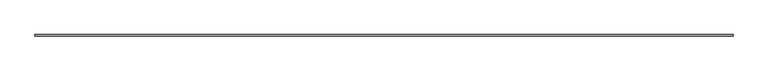
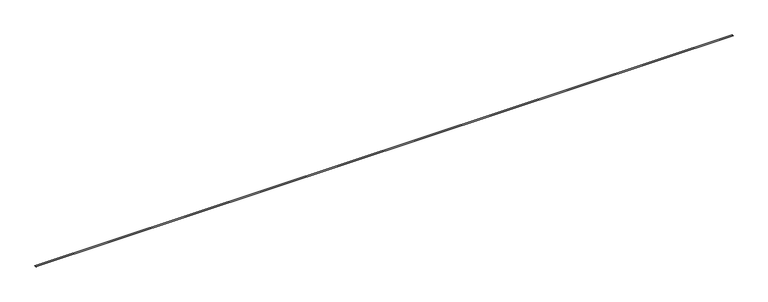
"""IFC4 building model written with IfcOpenShell, lengths in millimetres: proxy geometry, Generic Models 7:Generic Models 1:2:Generic Models 1:2 : Generic Models 7:Generic Models 1:337419:31 : Generic Models 7:Generic Models 1:2:Generic Models 1:2 : Generic Models 7:Generic Models 1:337419:306751."""

import ifcopenshell
import ifcopenshell.guid

model = None  # the IFC model being written
_history = None  # IfcOwnerHistory: only IFC2X3 demands one
_inside = {}  # id of a spatial element -> (the spatial element, [elements in it])
_under = {}  # id of a project, library or spatial element -> (it, [spatial elements below it])
_declared = {}  # id of a project -> (the project, [libraries it declares])
_typed = {}  # id of a type object -> (the type object, [elements of that type])
_made_of = {}  # id of a material, layer set ... -> (it, [elements and type objects made of it])


def new_model(schema):
    """Start an empty IFC model of exactly this schema.

    Asked for "IFC4X3", IfcOpenShell would pick the latest addendum, in which some entities
    have other attributes; the version numbers below select the first issue.
    IFC2X3 requires an IfcOwnerHistory on every rooted entity: one is made here for all.
    """
    global model, _history
    if schema == "IFC4X3":
        model = ifcopenshell.file(schema_version=(4, 3, 0, 0))
    else:
        model = ifcopenshell.file(schema=schema)
    _inside.clear()
    _under.clear()
    _declared.clear()
    _typed.clear()
    _made_of.clear()
    _history = None
    if model.schema == "IFC2X3":
        org = make("IfcOrganization", Name="unknown")
        user = make(
            "IfcPersonAndOrganization",
            ThePerson=make("IfcPerson", FamilyName="unknown"),
            TheOrganization=org,
        )
        app = make(
            "IfcApplication",
            ApplicationDeveloper=org,
            Version="unknown",
            ApplicationFullName="unknown",
            ApplicationIdentifier="unknown",
        )
        _history = make(
            "IfcOwnerHistory",
            OwningUser=user,
            OwningApplication=app,
            ChangeAction="ADDED",
            CreationDate=0,
        )
    return model


def make(cls, **values):
    """One entity of the class cls with the attributes given. An attribute that is None is left unset."""
    return model.create_entity(
        cls, **{name: value for name, value in values.items() if value is not None}
    )


def rooted(cls, **values):
    """An entity with a GlobalId (a new one), such as an element, a storey or a relation."""
    return make(cls, GlobalId=ifcopenshell.guid.new(), OwnerHistory=_history, **values)


def si_unit(unit_type, name, prefix=None):
    """IfcSIUnit, for example si_unit("LENGTHUNIT", "METRE", prefix="MILLI")."""
    return make("IfcSIUnit", UnitType=unit_type, Prefix=prefix, Name=name)


def assignment(units):
    """IfcUnitAssignment: the units of a project."""
    return None if units is None else make("IfcUnitAssignment", Units=units)


def point(xyz):
    """IfcCartesianPoint."""
    return None if xyz is None else make("IfcCartesianPoint", Coordinates=xyz)


def direction(xyz):
    """IfcDirection."""
    return None if xyz is None else make("IfcDirection", DirectionRatios=xyz)


def frame(location, z_axis=None, x_axis=None):
    """IfcAxis2Placement3D, a coordinate frame: its origin and axes. An axis left out is left unset."""
    return make(
        "IfcAxis2Placement3D",
        Location=point(location),
        Axis=direction(z_axis),
        RefDirection=direction(x_axis),
    )


def origin():
    """The frame at (0, 0, 0) with its axes left unset."""
    return frame((0.0, 0.0, 0.0))


def place(relative_to, where):
    """IfcLocalPlacement: puts the frame where relative to a parent placement (None: the world)."""
    return make(
        "IfcLocalPlacement", PlacementRelTo=relative_to, RelativePlacement=where
    )


def context(
    kind, dimensions, precision=None, world=None, true_north=None, identifier=None
):
    """IfcGeometricRepresentationContext, for example the 3D "Model" context."""
    return make(
        "IfcGeometricRepresentationContext",
        ContextIdentifier=identifier,
        ContextType=kind,
        CoordinateSpaceDimension=dimensions,
        Precision=precision,
        WorldCoordinateSystem=world,
        TrueNorth=true_north,
    )


def project(units=None, contexts=None):
    """IfcProject with its units and contexts."""
    return rooted(
        "IfcProject",
        Name="project",
        RepresentationContexts=contexts,
        UnitsInContext=assignment(units),
    )


def spatial(cls, under=None, at=None, **own):
    """A site, building, storey or space (cls), placed at a placement, below another one or the project."""
    s = rooted(cls, ObjectPlacement=at, **own)
    if under is not None:
        _under.setdefault(under.id(), (under, []))[1].append(s)
    return s


def polyline(points):
    """IfcPolyline through the points."""
    return make("IfcPolyline", Points=[point(p) for p in points])


def outline(outer, holes=None, kind="AREA"):
    """IfcArbitraryClosedProfileDef: a profile drawn as a closed curve; with holes, ...WithVoids."""
    if holes is None:
        return make("IfcArbitraryClosedProfileDef", ProfileType=kind, OuterCurve=outer)
    return make(
        "IfcArbitraryProfileDefWithVoids",
        ProfileType=kind,
        OuterCurve=outer,
        InnerCurves=holes,
    )


def extrude(swept, where, along, depth):
    """IfcExtrudedAreaSolid: the profile swept, set in the frame where, extruded along a direction by depth."""
    return make(
        "IfcExtrudedAreaSolid",
        SweptArea=swept,
        Position=where,
        ExtrudedDirection=direction(along),
        Depth=depth,
    )


def shape(context_of_items, identifier, shape_type, items):
    """IfcShapeRepresentation: the items that make up one representation, for example the "Body"."""
    return make(
        "IfcShapeRepresentation",
        ContextOfItems=context_of_items,
        RepresentationIdentifier=identifier,
        RepresentationType=shape_type,
        Items=items,
    )


def source(mapping_origin, context_of_items, identifier, shape_type, items):
    """IfcRepresentationMap: a shape defined once, which mapped items show again and again."""
    return make(
        "IfcRepresentationMap",
        MappingOrigin=mapping_origin,
        MappedRepresentation=shape(context_of_items, identifier, shape_type, items),
    )


def transform(
    local_origin,
    x_axis=None,
    y_axis=None,
    z_axis=None,
    scale=None,
    scale2=None,
    scale3=None,
    uniform=True,
):
    """IfcCartesianTransformationOperator3D, or its non-uniform kind. x_axis, y_axis, z_axis: its Axis1, 2, 3."""
    if uniform:
        return make(
            "IfcCartesianTransformationOperator3D",
            Axis1=direction(x_axis),
            Axis2=direction(y_axis),
            LocalOrigin=point(local_origin),
            Scale=scale,
            Axis3=direction(z_axis),
        )
    return make(
        "IfcCartesianTransformationOperator3DnonUniform",
        Axis1=direction(x_axis),
        Axis2=direction(y_axis),
        LocalOrigin=point(local_origin),
        Scale=scale,
        Axis3=direction(z_axis),
        Scale2=scale2,
        Scale3=scale3,
    )


def mapped(mapping_source, mapping_target):
    """IfcMappedItem: shows the shape of a source again, moved by a transform."""
    return make(
        "IfcMappedItem", MappingSource=mapping_source, MappingTarget=mapping_target
    )


def made_of(thing, what):
    """Note that an element or type object is made of a material, layer set ...; save() writes the relation."""
    if what is not None:
        _made_of.setdefault(what.id(), (what, []))[1].append(thing)
    return thing


def element(
    cls,
    number,
    at=None,
    inside=None,
    cuts=None,
    type_object=None,
    material=None,
    context=None,
    identifier="Body",
    shape_type=None,
    held_by="IfcProductDefinitionShape",
    body=None,
    shapes=None,
    **own,
):
    """One element of the class cls, such as IfcWall. Its Tag is "e" and its number.

    at: its placement. inside: the storey or other place that contains it. cuts: it is an
    opening in that element (IfcRelVoidsElement). A single representation is given by context,
    identifier, shape_type and body (its items); several are given by shapes. held_by: the class
    of the entity that holds the representations. save() writes the other relations.
    """
    e = rooted(cls, Tag="e%d" % number, ObjectPlacement=at, **own)
    if body is not None:
        shapes = [shape(context, identifier, shape_type, body)]
    if shapes is not None:
        e.Representation = make(held_by, Representations=shapes)
    if inside is not None:
        _inside.setdefault(inside.id(), (inside, []))[1].append(e)
    if cuts is not None:
        rooted(
            "IfcRelVoidsElement", RelatingBuildingElement=cuts, RelatedOpeningElement=e
        )
    if type_object is not None:
        _typed.setdefault(type_object.id(), (type_object, []))[1].append(e)
    return made_of(e, material)


def aggregate(whole, parts):
    """IfcRelAggregates: a whole, such as a stair, and the parts it consists of."""
    return rooted("IfcRelAggregates", RelatingObject=whole, RelatedObjects=parts)


def save(model, path):
    """Write the relations noted so far, then the file.

    IfcRelAggregates (storeys below a building ...), IfcRelContainedInSpatialStructure (elements
    in a storey), IfcRelDefinesByType, IfcRelAssociatesMaterial and IfcRelDeclares: one each for
    every whole, place, type object, material and project.
    """
    for whole, parts in _under.values():
        aggregate(whole, parts)
    for where, things in _inside.values():
        rooted(
            "IfcRelContainedInSpatialStructure",
            RelatedElements=things,
            RelatingStructure=where,
        )
    for kind, things in _typed.values():
        rooted("IfcRelDefinesByType", RelatedObjects=things, RelatingType=kind)
    for what, things in _made_of.values():
        rooted("IfcRelAssociatesMaterial", RelatedObjects=things, RelatingMaterial=what)
    for by, libraries in _declared.values():
        rooted("IfcRelDeclares", RelatingContext=by, RelatedDefinitions=libraries)
    model.write(path)


def generic_models_873e97bd(model_context):
    return source(origin(), model_context, "Body", "SweptSolid", [
        extrude(outline(polyline([(0.0, -164.8422109), (0.0, 0.0), (76200.0204281, 0.0), (76200.0204281, -164.8422109), (0.0, -164.8422109)])), frame((667506.057152, -567794.4782291, 8578.526715), z_axis=(0.0, -0.041630544767773385, 0.9991330730900356), x_axis=(-1.0, 0.0, 0.0)), (0.0, 0.0, 1.0), 12.7),
    ])


if __name__ == "__main__":
    model = new_model("IFC4")
    model_context = context("Model", 3, world=origin())
    ifc_project = project(units=[si_unit("LENGTHUNIT", "METRE", prefix="MILLI")], contexts=[model_context])
    site = spatial("IfcSite", under=ifc_project)
    building = spatial("IfcBuilding", under=site)
    placement = place(None, origin())
    generic_models_shape = generic_models_873e97bd(model_context)
    element("IfcBuildingElementProxy", 1, Name="Generic Models 7:Generic Models 1:2:Generic Models 1:2 : Generic Models 7:Generic Models 1:337419:31 : Generic Models 7:Generic Models 1:2:Generic Models 1:2 : Generic Models 7:Generic Models 1:337419:306751", ObjectType="Generic Models 7:Generic Models 1:2:Generic Models 1:2 : Generic Models 7:Generic Models 1:337419:31 : Generic Models 7:Generic Models 1:2:Generic Models 1:2 : Generic Models 7:Generic Models 1:337419:306751", at=placement, inside=building, context=model_context, shape_type="MappedRepresentation", body=[
        mapped(generic_models_shape, transform((0.0, 0.0, 0.0), x_axis=(1.0, 0.0, 0.0), y_axis=(0.0, 1.0, 0.0), z_axis=(0.0, 0.0, 1.0))),
    ])
    save(model, "model.ifc")

# Revit data of these elements
# Type "Generic Models 7:Generic Models 1:2:Generic Models 1:2 : Generic Models 7:Generic Models 1:337419:31 : Generic Models 7:Generic Models 1:2:Generic Models 1:2 : Generic Models 7:Generic Models 1:337419:306751"
#   NameOverride = "Generic Models 7:Generic Models 1:2:Generic Models 1:2 : Generic Models 7:Generic Models 1:337419:306751"
#   ObjectTypeOverride = "Generic Models 1:2 : Generic Models 7:Generic Models 1:337419"
#   Reference = "Generic Models 1"
#   Tag = "306751"
# Element 1 (IfcBuildingElementProxy, "Generic Models 7:Generic Models 1:2:Generic Models 1:2 : Generic Models 7:Generic Models 1:337419:31 : Generic Models 7:Generic Models 1:2:Generic Models 1:2 : Generic Models 7:Generic Models 1:337419:306751")
#   Materials on its faces: "FIRE RETARDTANT WOOD BLOCKING - SIZE AS NEC."
# Materials
#   "FIRE RETARDTANT WOOD BLOCKING - SIZE AS NEC.": class "Wood", colour RGB 144 113 62, transparency 0, Description = "Pinus Echinata", Cost = 0
